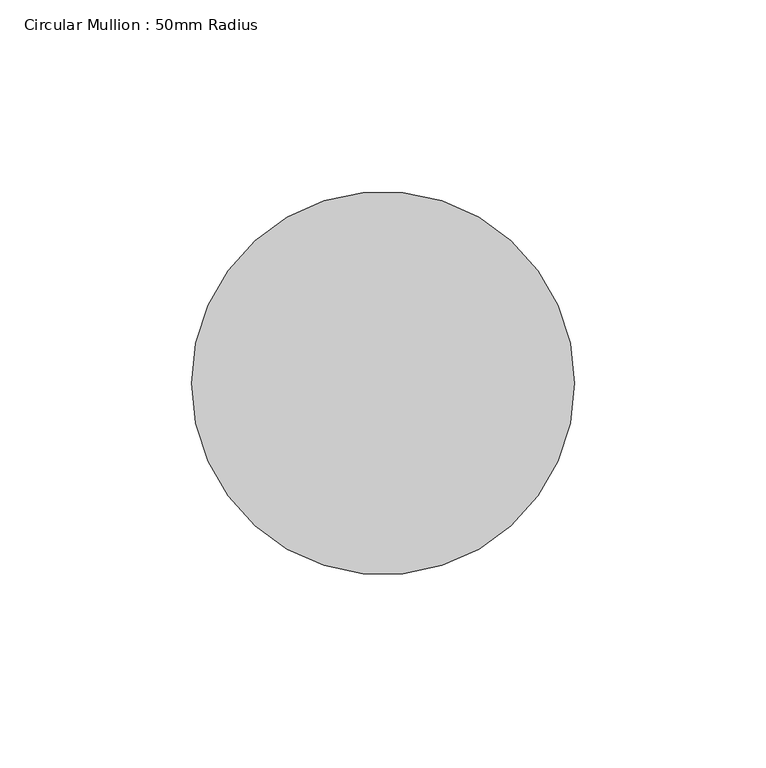
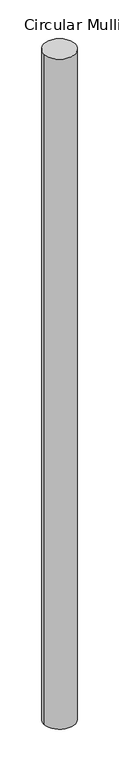
"""IFC4 building model written with IfcOpenShell, lengths in millimetres: member geometry, Circular Mullion : 50mm Radius."""

from ifc_helpers import new_model, si_unit, point, frame, origin, origin_2d, place, context, project, spatial, circle_curve, trimmed, segment, composite_curve, outline, extrude, source, transform, mapped, element, save


def circular_mullion_50mm_radius_6c88f229(model_context):
    return source(origin(), model_context, "Body", "SweptSolid", [
        extrude(outline(composite_curve([segment(trimmed(circle_curve(origin_2d(), 50.0), [point((50.0, 0.0))], [point((-50.0, 0.0))], False, "CARTESIAN"), True, "CONTINUOUS"), segment(trimmed(circle_curve(origin_2d(), 50.0), [point((-50.0, 0.0))], [point((50.0, 0.0))], False, "CARTESIAN"), True, "CONTINUOUS")], self_intersect=False)), frame((0.0, 0.0, -2274.851291), z_axis=(0.0, 0.0, 1.0), x_axis=(1.0, 0.0, 0.0)), (0.0, 0.0, 1.0), 2274.851291),
    ])


if __name__ == "__main__":
    model = new_model("IFC4")
    model_context = context("Model", 3, world=origin())
    ifc_project = project(units=[si_unit("LENGTHUNIT", "METRE", prefix="MILLI")], contexts=[model_context])
    site = spatial("IfcSite", under=ifc_project)
    building = spatial("IfcBuilding", under=site)
    placement = place(None, origin())
    circular_mullion_50mm_radius_shape = circular_mullion_50mm_radius_6c88f229(model_context)
    element("IfcMember", 1, ObjectType="Circular Mullion : 50mm Radius", at=placement, inside=building, context=model_context, shape_type="MappedRepresentation", body=[
        mapped(circular_mullion_50mm_radius_shape, transform((0.0, 0.0, 0.0), x_axis=(1.0, 0.0, 0.0), y_axis=(0.0, 1.0, 0.0), z_axis=(0.0, 0.0, 1.0))),
    ])
    save(model, "model.ifc")

# Revit data of these elements
# Type "Circular Mullion : 50mm Radius"
#   built-in parameter 1007350 = 0.164042 (stored number, unit not read)
# Element 1 (IfcMember, "Circular Mullion : 50mm Radius")
#   Materials on its faces: "Aluminium"
# Materials
#   "Aluminium": class "Metal", colour RGB 247 247 247, transparency 0, Description = "Aluminium 6061", Cost = 0
